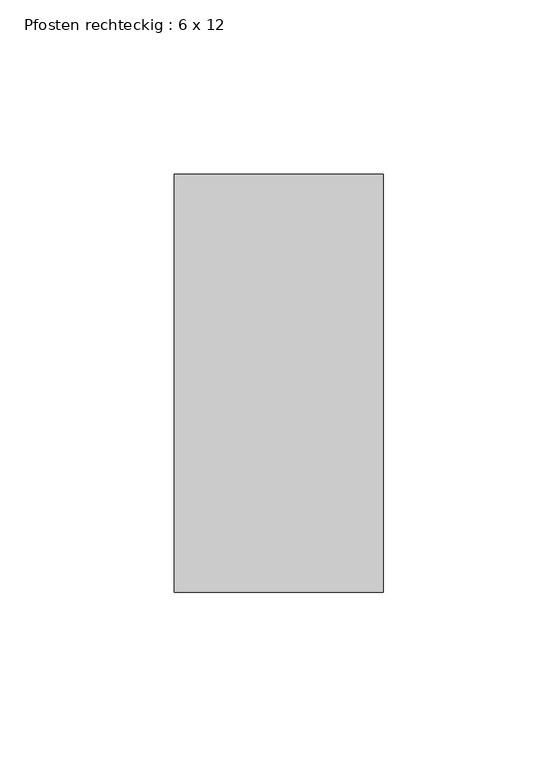
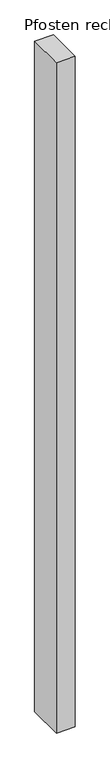
"""IFC4 building model written with IfcOpenShell, lengths in millimetres: member geometry, Pfosten rechteckig : 6 x 12."""

from ifc_helpers import new_model, si_unit, frame, origin, place, context, project, spatial, polyline, outline, extrude, source, transform, mapped, element, save


def pfosten_rechteckig_6_x_12_1a9f97fb(model_context):
    return source(origin(), model_context, "Body", "SweptSolid", [
        extrude(outline(polyline([(30.0, 60.0), (30.0, -60.0), (-30.0, -60.0), (-30.0, 60.0), (30.0, 60.0)])), frame((0.0, 0.0, -2267.088502), z_axis=(0.0, 0.0, 1.0), x_axis=(1.0, 0.0, 0.0)), (0.0, 0.0, 1.0), 2267.088502),
    ])


if __name__ == "__main__":
    model = new_model("IFC4")
    model_context = context("Model", 3, world=origin())
    ifc_project = project(units=[si_unit("LENGTHUNIT", "METRE", prefix="MILLI")], contexts=[model_context])
    site = spatial("IfcSite", under=ifc_project)
    building = spatial("IfcBuilding", under=site)
    placement = place(None, origin())
    pfosten_rechteckig_6_x_12_shape = pfosten_rechteckig_6_x_12_1a9f97fb(model_context)
    element("IfcMember", 1, ObjectType="Pfosten rechteckig : 6 x 12", at=placement, inside=building, context=model_context, shape_type="MappedRepresentation", body=[
        mapped(pfosten_rechteckig_6_x_12_shape, transform((0.0, 0.0, 0.0), x_axis=(1.0, 0.0, 0.0), y_axis=(0.0, 1.0, 0.0), z_axis=(0.0, 0.0, 1.0))),
    ])
    save(model, "model.ifc")

# Revit data of these elements
# Type "Pfosten rechteckig : 6 x 12"
#   built-in parameter 1007304 = 0.393701 (stored number, unit not read)
#   built-in parameter 1007301 = 0.0984252 (stored number, unit not read)
#   built-in parameter 1007300 = 0.0984252 (stored number, unit not read)
# Element 1 (IfcMember, "Pfosten rechteckig : 6 x 12")
#   Materials on its faces: "Metall - verzinkt"
# Materials
#   "Metall - verzinkt": class "Allgemeines", colour RGB 200 200 200, transparency 0, Cost = 0
